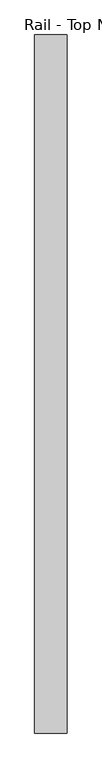
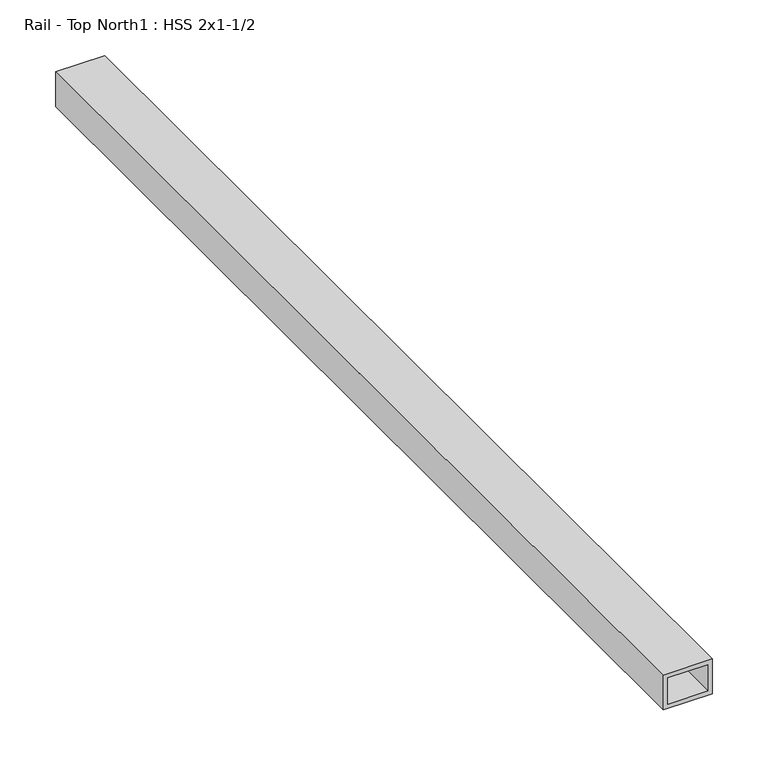
"""IFC4 building model written with IfcOpenShell, lengths in millimetres: proxy geometry, Rail - Top North1 : HSS 2x1-1/2."""

from ifc_helpers import new_model, si_unit, frame, origin, place, context, project, spatial, polyline, outline, extrude, source, transform, mapped, element, save


def rail_top_north1_hss_2x1_1_2_5f745a76(model_context):
    return source(origin(), model_context, "Body", "SweptSolid", [
        extrude(outline(polyline([(2400.3, 587416.6934739), (2438.4, 587416.6934739), (2438.4, 587365.8934739), (2400.3, 587365.8934739), (2400.3, 587416.6934739)]), holes=[polyline([(2433.6375, 587411.9309739), (2405.0625, 587411.9309739), (2405.0625, 587370.6559739), (2433.6375, 587370.6559739), (2433.6375, 587411.9309739)])]), frame((0.0, -535201.5663841, 0.0), z_axis=(0.0, 1.0, 0.0), x_axis=(0.0, 0.0, 1.0)), (0.0, 0.0, 1.0), 1092.2),
    ])


if __name__ == "__main__":
    model = new_model("IFC4")
    model_context = context("Model", 3, world=origin())
    ifc_project = project(units=[si_unit("LENGTHUNIT", "METRE", prefix="MILLI")], contexts=[model_context])
    site = spatial("IfcSite", under=ifc_project)
    building = spatial("IfcBuilding", under=site)
    placement = place(None, origin())
    rail_top_north1_hss_2x1_1_2_shape = rail_top_north1_hss_2x1_1_2_5f745a76(model_context)
    element("IfcBuildingElementProxy", 1, Name="Rail - Top North1 : HSS 2x1-1/2", ObjectType="Rail - Top North1 : HSS 2x1-1/2", at=placement, inside=building, context=model_context, shape_type="MappedRepresentation", body=[
        mapped(rail_top_north1_hss_2x1_1_2_shape, transform((0.0, 0.0, 0.0), x_axis=(1.0, 0.0, 0.0), y_axis=(0.0, 1.0, 0.0), z_axis=(0.0, 0.0, 1.0))),
    ])
    save(model, "model.ifc")

# Revit data of these elements
# Element 1 (IfcBuildingElementProxy, "Rail - Top North1 : HSS 2x1-1/2")
#   Materials on its faces: "1-1/2\"X2\" GALV. STL HSS TUBING"
# Materials
#   "1-1/2\"X2\" GALV. STL HSS TUBING": class "Generic", colour RGB 211 211 207, transparency 0, Cost = 0
